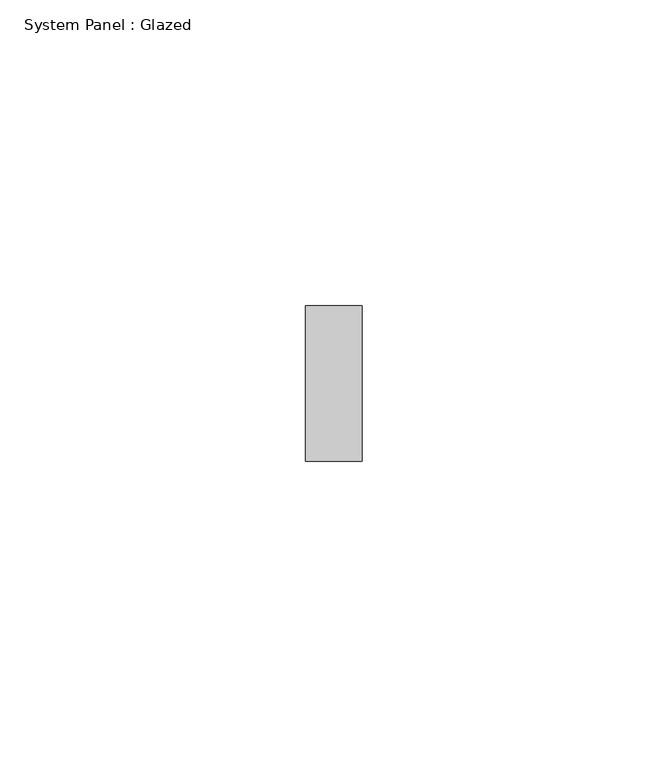
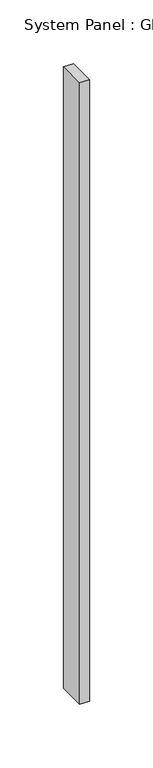
"""IFC4 building model written with IfcOpenShell, lengths in millimetres: plate geometry, System Panel : Glazed."""

import ifcopenshell
import ifcopenshell.guid

model = None  # the IFC model being written
_history = None  # IfcOwnerHistory: only IFC2X3 demands one
_inside = {}  # id of a spatial element -> (the spatial element, [elements in it])
_under = {}  # id of a project, library or spatial element -> (it, [spatial elements below it])
_declared = {}  # id of a project -> (the project, [libraries it declares])
_typed = {}  # id of a type object -> (the type object, [elements of that type])
_made_of = {}  # id of a material, layer set ... -> (it, [elements and type objects made of it])


def new_model(schema):
    """Start an empty IFC model of exactly this schema.

    Asked for "IFC4X3", IfcOpenShell would pick the latest addendum, in which some entities
    have other attributes; the version numbers below select the first issue.
    IFC2X3 requires an IfcOwnerHistory on every rooted entity: one is made here for all.
    """
    global model, _history
    if schema == "IFC4X3":
        model = ifcopenshell.file(schema_version=(4, 3, 0, 0))
    else:
        model = ifcopenshell.file(schema=schema)
    _inside.clear()
    _under.clear()
    _declared.clear()
    _typed.clear()
    _made_of.clear()
    _history = None
    if model.schema == "IFC2X3":
        org = make("IfcOrganization", Name="unknown")
        user = make(
            "IfcPersonAndOrganization",
            ThePerson=make("IfcPerson", FamilyName="unknown"),
            TheOrganization=org,
        )
        app = make(
            "IfcApplication",
            ApplicationDeveloper=org,
            Version="unknown",
            ApplicationFullName="unknown",
            ApplicationIdentifier="unknown",
        )
        _history = make(
            "IfcOwnerHistory",
            OwningUser=user,
            OwningApplication=app,
            ChangeAction="ADDED",
            CreationDate=0,
        )
    return model


def make(cls, **values):
    """One entity of the class cls with the attributes given. An attribute that is None is left unset."""
    return model.create_entity(
        cls, **{name: value for name, value in values.items() if value is not None}
    )


def rooted(cls, **values):
    """An entity with a GlobalId (a new one), such as an element, a storey or a relation."""
    return make(cls, GlobalId=ifcopenshell.guid.new(), OwnerHistory=_history, **values)


def si_unit(unit_type, name, prefix=None):
    """IfcSIUnit, for example si_unit("LENGTHUNIT", "METRE", prefix="MILLI")."""
    return make("IfcSIUnit", UnitType=unit_type, Prefix=prefix, Name=name)


def assignment(units):
    """IfcUnitAssignment: the units of a project."""
    return None if units is None else make("IfcUnitAssignment", Units=units)


def point(xyz):
    """IfcCartesianPoint."""
    return None if xyz is None else make("IfcCartesianPoint", Coordinates=xyz)


def direction(xyz):
    """IfcDirection."""
    return None if xyz is None else make("IfcDirection", DirectionRatios=xyz)


def frame(location, z_axis=None, x_axis=None):
    """IfcAxis2Placement3D, a coordinate frame: its origin and axes. An axis left out is left unset."""
    return make(
        "IfcAxis2Placement3D",
        Location=point(location),
        Axis=direction(z_axis),
        RefDirection=direction(x_axis),
    )


def origin():
    """The frame at (0, 0, 0) with its axes left unset."""
    return frame((0.0, 0.0, 0.0))


def origin_with_axes():
    """The frame at (0, 0, 0) with the z axis (0, 0, 1) and the x axis (1, 0, 0) written out."""
    return frame((0.0, 0.0, 0.0), z_axis=(0.0, 0.0, 1.0), x_axis=(1.0, 0.0, 0.0))


def place(relative_to, where):
    """IfcLocalPlacement: puts the frame where relative to a parent placement (None: the world)."""
    return make(
        "IfcLocalPlacement", PlacementRelTo=relative_to, RelativePlacement=where
    )


def context(
    kind, dimensions, precision=None, world=None, true_north=None, identifier=None
):
    """IfcGeometricRepresentationContext, for example the 3D "Model" context."""
    return make(
        "IfcGeometricRepresentationContext",
        ContextIdentifier=identifier,
        ContextType=kind,
        CoordinateSpaceDimension=dimensions,
        Precision=precision,
        WorldCoordinateSystem=world,
        TrueNorth=true_north,
    )


def project(units=None, contexts=None):
    """IfcProject with its units and contexts."""
    return rooted(
        "IfcProject",
        Name="project",
        RepresentationContexts=contexts,
        UnitsInContext=assignment(units),
    )


def spatial(cls, under=None, at=None, **own):
    """A site, building, storey or space (cls), placed at a placement, below another one or the project."""
    s = rooted(cls, ObjectPlacement=at, **own)
    if under is not None:
        _under.setdefault(under.id(), (under, []))[1].append(s)
    return s


def polyline(points):
    """IfcPolyline through the points."""
    return make("IfcPolyline", Points=[point(p) for p in points])


def outline(outer, holes=None, kind="AREA"):
    """IfcArbitraryClosedProfileDef: a profile drawn as a closed curve; with holes, ...WithVoids."""
    if holes is None:
        return make("IfcArbitraryClosedProfileDef", ProfileType=kind, OuterCurve=outer)
    return make(
        "IfcArbitraryProfileDefWithVoids",
        ProfileType=kind,
        OuterCurve=outer,
        InnerCurves=holes,
    )


def extrude(swept, where, along, depth):
    """IfcExtrudedAreaSolid: the profile swept, set in the frame where, extruded along a direction by depth."""
    return make(
        "IfcExtrudedAreaSolid",
        SweptArea=swept,
        Position=where,
        ExtrudedDirection=direction(along),
        Depth=depth,
    )


def shape(context_of_items, identifier, shape_type, items):
    """IfcShapeRepresentation: the items that make up one representation, for example the "Body"."""
    return make(
        "IfcShapeRepresentation",
        ContextOfItems=context_of_items,
        RepresentationIdentifier=identifier,
        RepresentationType=shape_type,
        Items=items,
    )


def source(mapping_origin, context_of_items, identifier, shape_type, items):
    """IfcRepresentationMap: a shape defined once, which mapped items show again and again."""
    return make(
        "IfcRepresentationMap",
        MappingOrigin=mapping_origin,
        MappedRepresentation=shape(context_of_items, identifier, shape_type, items),
    )


def transform(
    local_origin,
    x_axis=None,
    y_axis=None,
    z_axis=None,
    scale=None,
    scale2=None,
    scale3=None,
    uniform=True,
):
    """IfcCartesianTransformationOperator3D, or its non-uniform kind. x_axis, y_axis, z_axis: its Axis1, 2, 3."""
    if uniform:
        return make(
            "IfcCartesianTransformationOperator3D",
            Axis1=direction(x_axis),
            Axis2=direction(y_axis),
            LocalOrigin=point(local_origin),
            Scale=scale,
            Axis3=direction(z_axis),
        )
    return make(
        "IfcCartesianTransformationOperator3DnonUniform",
        Axis1=direction(x_axis),
        Axis2=direction(y_axis),
        LocalOrigin=point(local_origin),
        Scale=scale,
        Axis3=direction(z_axis),
        Scale2=scale2,
        Scale3=scale3,
    )


def mapped(mapping_source, mapping_target):
    """IfcMappedItem: shows the shape of a source again, moved by a transform."""
    return make(
        "IfcMappedItem", MappingSource=mapping_source, MappingTarget=mapping_target
    )


def made_of(thing, what):
    """Note that an element or type object is made of a material, layer set ...; save() writes the relation."""
    if what is not None:
        _made_of.setdefault(what.id(), (what, []))[1].append(thing)
    return thing


def element(
    cls,
    number,
    at=None,
    inside=None,
    cuts=None,
    type_object=None,
    material=None,
    context=None,
    identifier="Body",
    shape_type=None,
    held_by="IfcProductDefinitionShape",
    body=None,
    shapes=None,
    **own,
):
    """One element of the class cls, such as IfcWall. Its Tag is "e" and its number.

    at: its placement. inside: the storey or other place that contains it. cuts: it is an
    opening in that element (IfcRelVoidsElement). A single representation is given by context,
    identifier, shape_type and body (its items); several are given by shapes. held_by: the class
    of the entity that holds the representations. save() writes the other relations.
    """
    e = rooted(cls, Tag="e%d" % number, ObjectPlacement=at, **own)
    if body is not None:
        shapes = [shape(context, identifier, shape_type, body)]
    if shapes is not None:
        e.Representation = make(held_by, Representations=shapes)
    if inside is not None:
        _inside.setdefault(inside.id(), (inside, []))[1].append(e)
    if cuts is not None:
        rooted(
            "IfcRelVoidsElement", RelatingBuildingElement=cuts, RelatedOpeningElement=e
        )
    if type_object is not None:
        _typed.setdefault(type_object.id(), (type_object, []))[1].append(e)
    return made_of(e, material)


def aggregate(whole, parts):
    """IfcRelAggregates: a whole, such as a stair, and the parts it consists of."""
    return rooted("IfcRelAggregates", RelatingObject=whole, RelatedObjects=parts)


def save(model, path):
    """Write the relations noted so far, then the file.

    IfcRelAggregates (storeys below a building ...), IfcRelContainedInSpatialStructure (elements
    in a storey), IfcRelDefinesByType, IfcRelAssociatesMaterial and IfcRelDeclares: one each for
    every whole, place, type object, material and project.
    """
    for whole, parts in _under.values():
        aggregate(whole, parts)
    for where, things in _inside.values():
        rooted(
            "IfcRelContainedInSpatialStructure",
            RelatedElements=things,
            RelatingStructure=where,
        )
    for kind, things in _typed.values():
        rooted("IfcRelDefinesByType", RelatedObjects=things, RelatingType=kind)
    for what, things in _made_of.values():
        rooted("IfcRelAssociatesMaterial", RelatedObjects=things, RelatingMaterial=what)
    for by, libraries in _declared.values():
        rooted("IfcRelDeclares", RelatingContext=by, RelatedDefinitions=libraries)
    model.write(path)


def system_panel_glazed_8e796718(model_context):
    return source(origin(), model_context, "Body", "SweptSolid", [
        extrude(outline(polyline([(4.6013366, 19.05), (-4.6013366, 19.05), (-4.6013366, 44.45), (4.6013366, 44.45), (4.6013366, 19.05)])), origin_with_axes(), (0.0, 0.0, 1.0), 596.9),
    ])


if __name__ == "__main__":
    model = new_model("IFC4")
    model_context = context("Model", 3, world=origin())
    ifc_project = project(units=[si_unit("LENGTHUNIT", "METRE", prefix="MILLI")], contexts=[model_context])
    site = spatial("IfcSite", under=ifc_project)
    building = spatial("IfcBuilding", under=site)
    placement = place(None, origin())
    system_panel_glazed_shape = system_panel_glazed_8e796718(model_context)
    element("IfcPlate", 1, ObjectType="System Panel : Glazed", at=placement, inside=building, context=model_context, shape_type="MappedRepresentation", body=[
        mapped(system_panel_glazed_shape, transform((0.0, 0.0, 0.0), x_axis=(1.0, 0.0, 0.0), y_axis=(0.0, 1.0, 0.0), z_axis=(0.0, 0.0, 1.0))),
    ])
    save(model, "model.ifc")

# Revit data of these elements
# Element 1 (IfcPlate, "System Panel : Glazed")
#   Materials on its faces: "Glass"
# Materials
#   "Glass": class "Glass", colour RGB 0 128 192, transparency 0.75
